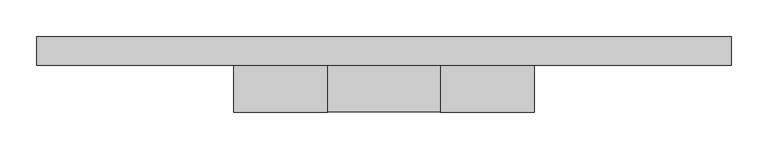
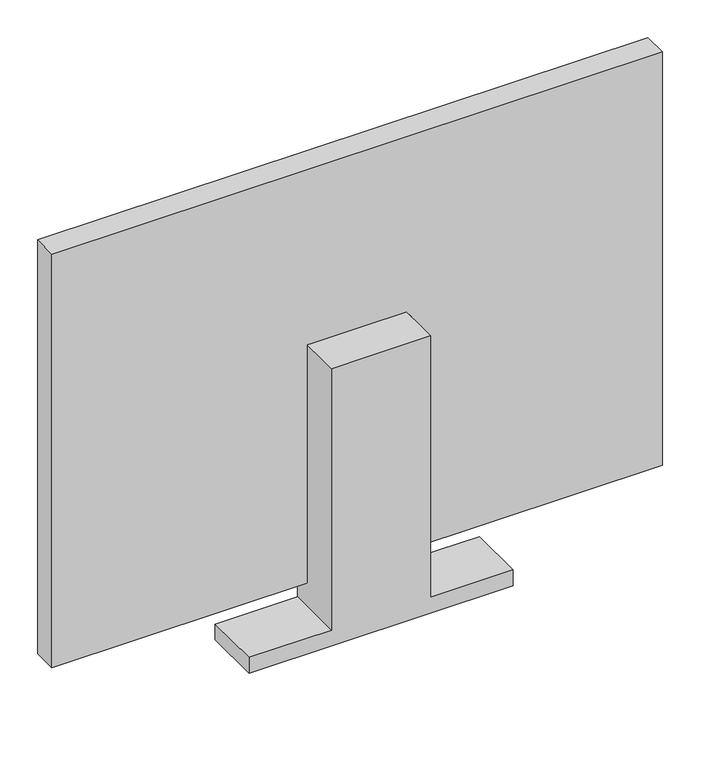
"""IFC4 building model written with IfcOpenShell, lengths in millimetres: proxy geometry, TV - NON-COLLECTUS : -."""

from ifc_helpers import new_model, si_unit, frame, origin, place, context, project, spatial, polyline, outline, extrude, source, transform, mapped, element, save


def specialty_equipment_b8060523(model_context):
    return source(origin(), model_context, "Body", "SweptSolid", [
        extrude(outline(polyline([(450.799327, 76.2), (450.799327, -76.2), (25.4, -76.2), (25.4, -203.2), (0.0, -203.2), (0.0, 203.2), (25.4, 203.2), (25.4, 76.2), (450.799327, 76.2)])), frame((0.0, -63.5, 0.0), z_axis=(0.0, 1.0, 0.0), x_axis=(0.0, 0.0, 1.0)), (0.0, 0.0, 1.0), 89.6753219),
        extrude(outline(polyline([(76.2, 0.0), (76.2, -12.7), (-76.2, -12.7), (-76.2, 0.0), (76.2, 0.0)])), frame((0.0, 0.0, 349.199327), z_axis=(0.0, 0.0, 1.0), x_axis=(1.0, 0.0, 0.0)), (0.0, 0.0, 1.0), 101.6),
        extrude(outline(polyline([(469.99906, 0.0), (-469.99906, 0.0), (-469.99906, 38.1), (469.99906, 38.1), (469.99906, 0.0)])), frame((0.0, 0.0, 63.5), z_axis=(0.0, 0.0, 1.0), x_axis=(1.0, 0.0, 0.0)), (0.0, 0.0, 1.0), 672.998654),
    ])


if __name__ == "__main__":
    model = new_model("IFC4")
    model_context = context("Model", 3, world=origin())
    ifc_project = project(units=[si_unit("LENGTHUNIT", "METRE", prefix="MILLI")], contexts=[model_context])
    site = spatial("IfcSite", under=ifc_project)
    building = spatial("IfcBuilding", under=site)
    placement = place(None, origin())
    specialty_equipment_shape = specialty_equipment_b8060523(model_context)
    element("IfcBuildingElementProxy", 1, Name="TV - NON-COLLECTUS : -", ObjectType="TV - NON-COLLECTUS : -", at=placement, inside=building, context=model_context, shape_type="MappedRepresentation", body=[
        mapped(specialty_equipment_shape, transform((0.0, 0.0, 0.0), x_axis=(1.0, 0.0, 0.0), y_axis=(0.0, 1.0, 0.0), z_axis=(0.0, 0.0, 1.0))),
    ])
    save(model, "model.ifc")

# Revit data of these elements
# Type "TV - NON-COLLECTUS : -"
#   External ID [instance default] = ""
#   Width = 939.998 mm
#   Height = 672.999 mm
#   Depth = 102 mm
#   Material = Light Grey
#   Default Elevation = 0
# Element 1 (IfcBuildingElementProxy, "TV - NON-COLLECTUS : -")
#   Materials on its faces: "Light Grey"
# Materials
#   "Light Grey": class "Generic", colour RGB 215 215 215, transparency 0, Cost = 0
